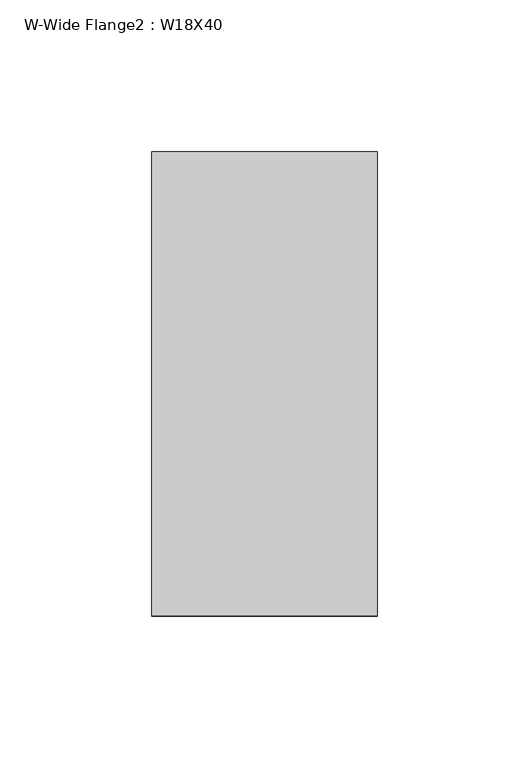
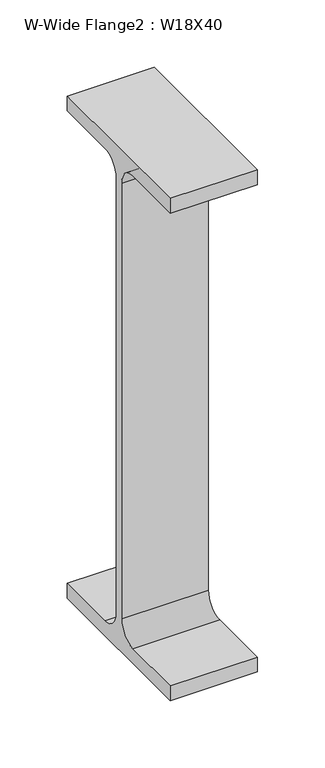
"""IFC4 building model written with IfcOpenShell, lengths in millimetres: beam geometry, W-Wide Flange2 : W18X40."""

from ifc_helpers import new_model, si_unit, point, frame, frame_2d, origin, place, context, project, spatial, polyline, circle_curve, trimmed, segment, composite_curve, outline, extrude, source, transform, mapped, element, save


def w_wide_flange2_w18x40_4655c839(model_context):
    return source(origin(), model_context, "Body", "SweptSolid", [
        extrude(outline(composite_curve([segment(polyline([(76.454, -213.995), (76.454, -227.33), (-76.454, -227.33), (-76.454, -213.995), (-20.828, -213.995)]), True, "CONTINUOUS"), segment(trimmed(circle_curve(frame_2d((-20.828, -197.1675)), 16.8275), [point((-20.828, -213.995))], [point((-4.0005, -197.1675))], True, "CARTESIAN"), True, "CONTINUOUS"), segment(polyline([(-4.0005, -197.1675), (-4.0005, 197.1675)]), True, "CONTINUOUS"), segment(trimmed(circle_curve(frame_2d((-20.828, 197.1675)), 16.8275), [point((-4.0005, 197.1675))], [point((-20.828, 213.995))], True, "CARTESIAN"), True, "CONTINUOUS"), segment(polyline([(-20.828, 213.995), (-76.454, 213.995), (-76.454, 227.33), (76.454, 227.33), (76.454, 213.995), (20.828, 213.995)]), True, "CONTINUOUS"), segment(trimmed(circle_curve(frame_2d((20.828, 197.1675)), 16.8275), [point((20.828, 213.995))], [point((4.0005, 197.1675))], True, "CARTESIAN"), True, "CONTINUOUS"), segment(polyline([(4.0005, 197.1675), (4.0005, -197.1675)]), True, "CONTINUOUS"), segment(trimmed(circle_curve(frame_2d((20.828, -197.1675)), 16.8275), [point((4.0005, -197.1675))], [point((20.828, -213.995))], True, "CARTESIAN"), True, "CONTINUOUS"), segment(polyline([(20.828, -213.995), (76.454, -213.995)]), True, "CONTINUOUS")], self_intersect=False)), frame((-68.2625, 0.0, 0.0), z_axis=(1.0, 0.0, 0.0), x_axis=(0.0, 1.0, 0.0)), (0.0, 0.0, 1.0), 74.215625),
    ])


if __name__ == "__main__":
    model = new_model("IFC4")
    model_context = context("Model", 3, world=origin())
    ifc_project = project(units=[si_unit("LENGTHUNIT", "METRE", prefix="MILLI")], contexts=[model_context])
    site = spatial("IfcSite", under=ifc_project)
    building = spatial("IfcBuilding", under=site)
    placement = place(None, origin())
    w_wide_flange2_w18x40_shape = w_wide_flange2_w18x40_4655c839(model_context)
    element("IfcBeam", 1, ObjectType="W-Wide Flange2 : W18X40", at=placement, inside=building, context=model_context, shape_type="MappedRepresentation", body=[
        mapped(w_wide_flange2_w18x40_shape, transform((0.0, 0.0, 0.0), x_axis=(1.0, 0.0, 0.0), y_axis=(0.0, 1.0, 0.0), z_axis=(0.0, 0.0, 1.0))),
    ])
    save(model, "model.ifc")

# Revit data of these elements
# Type "W-Wide Flange2 : W18X40"
#   Assembly Code = "B10"
#   W = 40
#   Length [instance default] = 5' - 0"
#   bf = 0' - 6.02"
#   d = 1' - 5.9"
#   k = 0' - 1 3/16"
#   k2 = 0' - 0.6625"
#   tf = 0' - 0.525"
#   tw = 0' - 0.315"
#   A = 0.0819444 SF
#   Structural Material [instance default] = Steel ASTM A992
# Element 1 (IfcBeam, "W-Wide Flange2 : W18X40")
#   Materials on its faces: "Steel ASTM A992"
# Materials
#   "Steel ASTM A992": class "Metal", colour RGB 199 199 199, transparency 0, Description = "Structural steel 50ksi", Cost = 0
